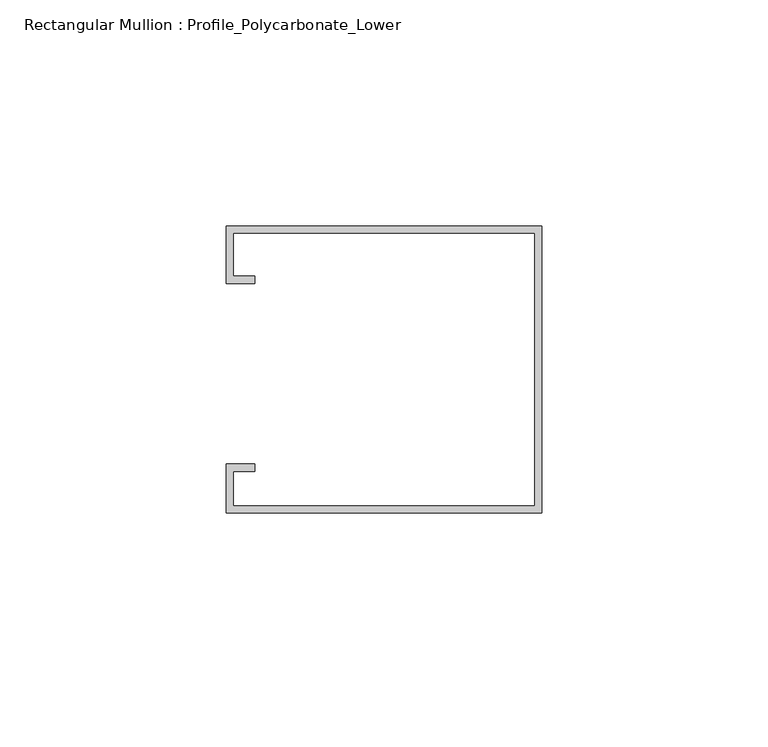
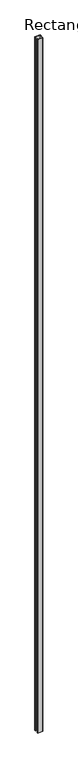
"""IFC4 building model written with IfcOpenShell, lengths in millimetres: member geometry, Rectangular Mullion : Profile_Polycarbonate_Lower."""

import ifcopenshell
import ifcopenshell.guid

model = None  # the IFC model being written
_history = None  # IfcOwnerHistory: only IFC2X3 demands one
_inside = {}  # id of a spatial element -> (the spatial element, [elements in it])
_under = {}  # id of a project, library or spatial element -> (it, [spatial elements below it])
_declared = {}  # id of a project -> (the project, [libraries it declares])
_typed = {}  # id of a type object -> (the type object, [elements of that type])
_made_of = {}  # id of a material, layer set ... -> (it, [elements and type objects made of it])


def new_model(schema):
    """Start an empty IFC model of exactly this schema.

    Asked for "IFC4X3", IfcOpenShell would pick the latest addendum, in which some entities
    have other attributes; the version numbers below select the first issue.
    IFC2X3 requires an IfcOwnerHistory on every rooted entity: one is made here for all.
    """
    global model, _history
    if schema == "IFC4X3":
        model = ifcopenshell.file(schema_version=(4, 3, 0, 0))
    else:
        model = ifcopenshell.file(schema=schema)
    _inside.clear()
    _under.clear()
    _declared.clear()
    _typed.clear()
    _made_of.clear()
    _history = None
    if model.schema == "IFC2X3":
        org = make("IfcOrganization", Name="unknown")
        user = make(
            "IfcPersonAndOrganization",
            ThePerson=make("IfcPerson", FamilyName="unknown"),
            TheOrganization=org,
        )
        app = make(
            "IfcApplication",
            ApplicationDeveloper=org,
            Version="unknown",
            ApplicationFullName="unknown",
            ApplicationIdentifier="unknown",
        )
        _history = make(
            "IfcOwnerHistory",
            OwningUser=user,
            OwningApplication=app,
            ChangeAction="ADDED",
            CreationDate=0,
        )
    return model


def make(cls, **values):
    """One entity of the class cls with the attributes given. An attribute that is None is left unset."""
    return model.create_entity(
        cls, **{name: value for name, value in values.items() if value is not None}
    )


def rooted(cls, **values):
    """An entity with a GlobalId (a new one), such as an element, a storey or a relation."""
    return make(cls, GlobalId=ifcopenshell.guid.new(), OwnerHistory=_history, **values)


def si_unit(unit_type, name, prefix=None):
    """IfcSIUnit, for example si_unit("LENGTHUNIT", "METRE", prefix="MILLI")."""
    return make("IfcSIUnit", UnitType=unit_type, Prefix=prefix, Name=name)


def assignment(units):
    """IfcUnitAssignment: the units of a project."""
    return None if units is None else make("IfcUnitAssignment", Units=units)


def point(xyz):
    """IfcCartesianPoint."""
    return None if xyz is None else make("IfcCartesianPoint", Coordinates=xyz)


def direction(xyz):
    """IfcDirection."""
    return None if xyz is None else make("IfcDirection", DirectionRatios=xyz)


def frame(location, z_axis=None, x_axis=None):
    """IfcAxis2Placement3D, a coordinate frame: its origin and axes. An axis left out is left unset."""
    return make(
        "IfcAxis2Placement3D",
        Location=point(location),
        Axis=direction(z_axis),
        RefDirection=direction(x_axis),
    )


def origin():
    """The frame at (0, 0, 0) with its axes left unset."""
    return frame((0.0, 0.0, 0.0))


def place(relative_to, where):
    """IfcLocalPlacement: puts the frame where relative to a parent placement (None: the world)."""
    return make(
        "IfcLocalPlacement", PlacementRelTo=relative_to, RelativePlacement=where
    )


def context(
    kind, dimensions, precision=None, world=None, true_north=None, identifier=None
):
    """IfcGeometricRepresentationContext, for example the 3D "Model" context."""
    return make(
        "IfcGeometricRepresentationContext",
        ContextIdentifier=identifier,
        ContextType=kind,
        CoordinateSpaceDimension=dimensions,
        Precision=precision,
        WorldCoordinateSystem=world,
        TrueNorth=true_north,
    )


def project(units=None, contexts=None):
    """IfcProject with its units and contexts."""
    return rooted(
        "IfcProject",
        Name="project",
        RepresentationContexts=contexts,
        UnitsInContext=assignment(units),
    )


def spatial(cls, under=None, at=None, **own):
    """A site, building, storey or space (cls), placed at a placement, below another one or the project."""
    s = rooted(cls, ObjectPlacement=at, **own)
    if under is not None:
        _under.setdefault(under.id(), (under, []))[1].append(s)
    return s


def polyline(points):
    """IfcPolyline through the points."""
    return make("IfcPolyline", Points=[point(p) for p in points])


def outline(outer, holes=None, kind="AREA"):
    """IfcArbitraryClosedProfileDef: a profile drawn as a closed curve; with holes, ...WithVoids."""
    if holes is None:
        return make("IfcArbitraryClosedProfileDef", ProfileType=kind, OuterCurve=outer)
    return make(
        "IfcArbitraryProfileDefWithVoids",
        ProfileType=kind,
        OuterCurve=outer,
        InnerCurves=holes,
    )


def extrude(swept, where, along, depth):
    """IfcExtrudedAreaSolid: the profile swept, set in the frame where, extruded along a direction by depth."""
    return make(
        "IfcExtrudedAreaSolid",
        SweptArea=swept,
        Position=where,
        ExtrudedDirection=direction(along),
        Depth=depth,
    )


def shape(context_of_items, identifier, shape_type, items):
    """IfcShapeRepresentation: the items that make up one representation, for example the "Body"."""
    return make(
        "IfcShapeRepresentation",
        ContextOfItems=context_of_items,
        RepresentationIdentifier=identifier,
        RepresentationType=shape_type,
        Items=items,
    )


def source(mapping_origin, context_of_items, identifier, shape_type, items):
    """IfcRepresentationMap: a shape defined once, which mapped items show again and again."""
    return make(
        "IfcRepresentationMap",
        MappingOrigin=mapping_origin,
        MappedRepresentation=shape(context_of_items, identifier, shape_type, items),
    )


def transform(
    local_origin,
    x_axis=None,
    y_axis=None,
    z_axis=None,
    scale=None,
    scale2=None,
    scale3=None,
    uniform=True,
):
    """IfcCartesianTransformationOperator3D, or its non-uniform kind. x_axis, y_axis, z_axis: its Axis1, 2, 3."""
    if uniform:
        return make(
            "IfcCartesianTransformationOperator3D",
            Axis1=direction(x_axis),
            Axis2=direction(y_axis),
            LocalOrigin=point(local_origin),
            Scale=scale,
            Axis3=direction(z_axis),
        )
    return make(
        "IfcCartesianTransformationOperator3DnonUniform",
        Axis1=direction(x_axis),
        Axis2=direction(y_axis),
        LocalOrigin=point(local_origin),
        Scale=scale,
        Axis3=direction(z_axis),
        Scale2=scale2,
        Scale3=scale3,
    )


def mapped(mapping_source, mapping_target):
    """IfcMappedItem: shows the shape of a source again, moved by a transform."""
    return make(
        "IfcMappedItem", MappingSource=mapping_source, MappingTarget=mapping_target
    )


def made_of(thing, what):
    """Note that an element or type object is made of a material, layer set ...; save() writes the relation."""
    if what is not None:
        _made_of.setdefault(what.id(), (what, []))[1].append(thing)
    return thing


def element(
    cls,
    number,
    at=None,
    inside=None,
    cuts=None,
    type_object=None,
    material=None,
    context=None,
    identifier="Body",
    shape_type=None,
    held_by="IfcProductDefinitionShape",
    body=None,
    shapes=None,
    **own,
):
    """One element of the class cls, such as IfcWall. Its Tag is "e" and its number.

    at: its placement. inside: the storey or other place that contains it. cuts: it is an
    opening in that element (IfcRelVoidsElement). A single representation is given by context,
    identifier, shape_type and body (its items); several are given by shapes. held_by: the class
    of the entity that holds the representations. save() writes the other relations.
    """
    e = rooted(cls, Tag="e%d" % number, ObjectPlacement=at, **own)
    if body is not None:
        shapes = [shape(context, identifier, shape_type, body)]
    if shapes is not None:
        e.Representation = make(held_by, Representations=shapes)
    if inside is not None:
        _inside.setdefault(inside.id(), (inside, []))[1].append(e)
    if cuts is not None:
        rooted(
            "IfcRelVoidsElement", RelatingBuildingElement=cuts, RelatedOpeningElement=e
        )
    if type_object is not None:
        _typed.setdefault(type_object.id(), (type_object, []))[1].append(e)
    return made_of(e, material)


def aggregate(whole, parts):
    """IfcRelAggregates: a whole, such as a stair, and the parts it consists of."""
    return rooted("IfcRelAggregates", RelatingObject=whole, RelatedObjects=parts)


def save(model, path):
    """Write the relations noted so far, then the file.

    IfcRelAggregates (storeys below a building ...), IfcRelContainedInSpatialStructure (elements
    in a storey), IfcRelDefinesByType, IfcRelAssociatesMaterial and IfcRelDeclares: one each for
    every whole, place, type object, material and project.
    """
    for whole, parts in _under.values():
        aggregate(whole, parts)
    for where, things in _inside.values():
        rooted(
            "IfcRelContainedInSpatialStructure",
            RelatedElements=things,
            RelatingStructure=where,
        )
    for kind, things in _typed.values():
        rooted("IfcRelDefinesByType", RelatedObjects=things, RelatingType=kind)
    for what, things in _made_of.values():
        rooted("IfcRelAssociatesMaterial", RelatedObjects=things, RelatingMaterial=what)
    for by, libraries in _declared.values():
        rooted("IfcRelDeclares", RelatingContext=by, RelatedDefinitions=libraries)
    model.write(path)


def rectangular_mullion_profile_polycarbonate_lower_4c106b6d(model_context):
    return source(origin(), model_context, "Body", "SweptSolid", [
        extrude(outline(polyline([(0.0, 32.7), (0.0, -30.8), (-69.85, -30.8), (-69.85, -20.0), (-63.5, -20.0), (-63.5, -21.5875), (-68.2625, -21.5875), (-68.2625, -29.2125), (-1.5875, -29.2125), (-1.5875, 31.1125), (-68.2625, 31.1125), (-68.2625, 21.5875), (-63.5, 21.5875), (-63.5, 20.0), (-69.85, 20.0), (-69.85, 32.7), (0.0, 32.7)])), frame((0.0, 0.0, -9907.5875), z_axis=(0.0, 0.0, 1.0), x_axis=(1.0, 0.0, 0.0)), (0.0, 0.0, 1.0), 9907.5875),
    ])


if __name__ == "__main__":
    model = new_model("IFC4")
    model_context = context("Model", 3, world=origin())
    ifc_project = project(units=[si_unit("LENGTHUNIT", "METRE", prefix="MILLI")], contexts=[model_context])
    site = spatial("IfcSite", under=ifc_project)
    building = spatial("IfcBuilding", under=site)
    placement = place(None, origin())
    rectangular_mullion_profile_polycarbonate_lower_shape = rectangular_mullion_profile_polycarbonate_lower_4c106b6d(model_context)
    element("IfcMember", 1, ObjectType="Rectangular Mullion : Profile_Polycarbonate_Lower", at=placement, inside=building, context=model_context, shape_type="MappedRepresentation", body=[
        mapped(rectangular_mullion_profile_polycarbonate_lower_shape, transform((0.0, 0.0, 0.0), x_axis=(1.0, 0.0, 0.0), y_axis=(0.0, 1.0, 0.0), z_axis=(0.0, 0.0, 1.0))),
    ])
    save(model, "model.ifc")

# Revit data of these elements
# Project information
#   Project Issue Date = "07/20/2015"
#   Project Status = "Project Status"
#   Client Name = "Xcel"
#   Project Address = "Enter address here"
#   Project Name = "Xcel Sports Complex"
#   Project Number = "Project Number"
# Type "Rectangular Mullion : Profile_Polycarbonate_Lower"
#   built-in parameter 1007322 = 0.208333 (stored number, unit not read)
#   built-in parameter 1007321 = 0 (stored number, unit not read)
#   built-in parameter 1007320 = 0.00520833 (stored number, unit not read)
